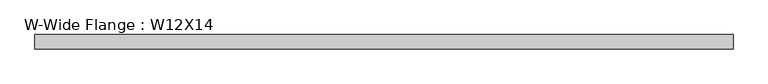
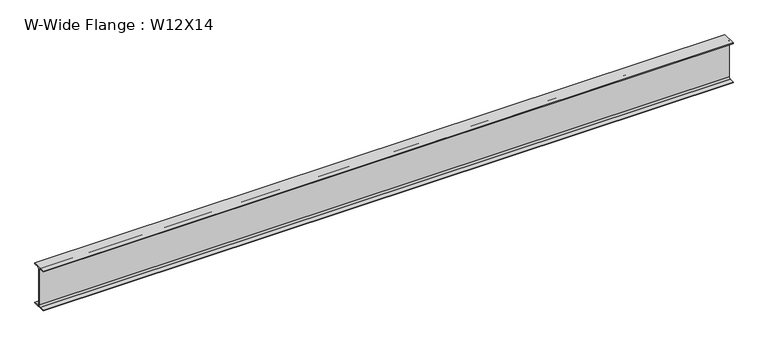
"""IFC4 building model written with IfcOpenShell, lengths in millimetres: beam geometry, W-Wide Flange : W12X14."""

from ifc_helpers import new_model, si_unit, point, frame, frame_2d, origin, place, context, project, spatial, polyline, circle_curve, trimmed, segment, composite_curve, outline, extrude, source, transform, mapped, element, save


def w_wide_flange_w12x14_1ca5f06a(model_context):
    return source(origin(), model_context, "Body", "SweptSolid", [
        extrude(outline(composite_curve([segment(polyline([(50.419, -145.415), (50.419, -151.13), (-50.419, -151.13), (-50.419, -145.415), (-15.875, -145.415)]), True, "CONTINUOUS"), segment(trimmed(circle_curve(frame_2d((-15.875, -132.08)), 13.335), [point((-15.875, -145.415))], [point((-2.54, -132.08))], True, "CARTESIAN"), True, "CONTINUOUS"), segment(polyline([(-2.54, -132.08), (-2.54, 132.08)]), True, "CONTINUOUS"), segment(trimmed(circle_curve(frame_2d((-15.875, 132.08)), 13.335), [point((-2.54, 132.08))], [point((-15.875, 145.415))], True, "CARTESIAN"), True, "CONTINUOUS"), segment(polyline([(-15.875, 145.415), (-50.419, 145.415), (-50.419, 151.13), (50.419, 151.13), (50.419, 145.415), (15.875, 145.415)]), True, "CONTINUOUS"), segment(trimmed(circle_curve(frame_2d((15.875, 132.08)), 13.335), [point((15.875, 145.415))], [point((2.54, 132.08))], True, "CARTESIAN"), True, "CONTINUOUS"), segment(polyline([(2.54, 132.08), (2.54, -132.08)]), True, "CONTINUOUS"), segment(trimmed(circle_curve(frame_2d((15.875, -132.08)), 13.335), [point((2.54, -132.08))], [point((15.875, -145.415))], True, "CARTESIAN"), True, "CONTINUOUS"), segment(polyline([(15.875, -145.415), (50.419, -145.415)]), True, "CONTINUOUS")], self_intersect=False)), frame((-2475.992, 0.0, 0.0), z_axis=(1.0, 0.0, 0.0), x_axis=(0.0, 1.0, 0.0)), (0.0, 0.0, 1.0), 4940.3),
    ])


if __name__ == "__main__":
    model = new_model("IFC4")
    model_context = context("Model", 3, world=origin())
    ifc_project = project(units=[si_unit("LENGTHUNIT", "METRE", prefix="MILLI")], contexts=[model_context])
    site = spatial("IfcSite", under=ifc_project)
    building = spatial("IfcBuilding", under=site)
    placement = place(None, origin())
    w_wide_flange_w12x14_shape = w_wide_flange_w12x14_1ca5f06a(model_context)
    element("IfcBeam", 1, ObjectType="W-Wide Flange : W12X14", at=placement, inside=building, context=model_context, shape_type="MappedRepresentation", body=[
        mapped(w_wide_flange_w12x14_shape, transform((0.0, 0.0, 0.0), x_axis=(1.0, 0.0, 0.0), y_axis=(0.0, 1.0, 0.0), z_axis=(0.0, 0.0, 1.0))),
    ])
    save(model, "model.ifc")

# Revit data of these elements
# Type "W-Wide Flange : W12X14"
#   Assembly Code = "B10"
#   W = 14
#   Length [instance default] = 5' - 0"
#   bf = 0' - 3.97"
#   d = 0' - 11.9"
#   k = 0' - 0 3/4"
#   k2 = 0' - 0.525"
#   tf = 0' - 0.225"
#   tw = 0' - 0.2"
#   A = 0.0288889 SF
#   Structural Material [instance default] = Steel ASTM A992
# Element 1 (IfcBeam, "W-Wide Flange : W12X14")
#   Materials on its faces: "Steel ASTM A992"
# Materials
#   "Steel ASTM A992": class "Metal", colour RGB 199 199 199, transparency 0, Description = "Structural steel 50ksi", Cost = 0
